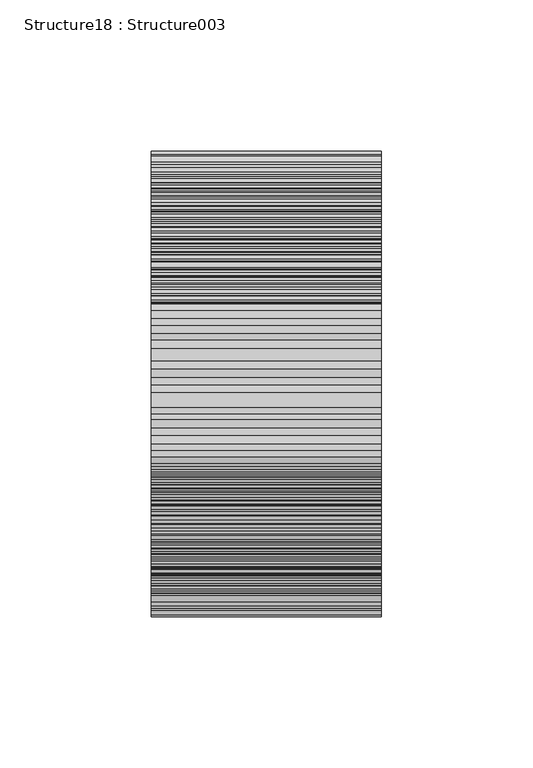
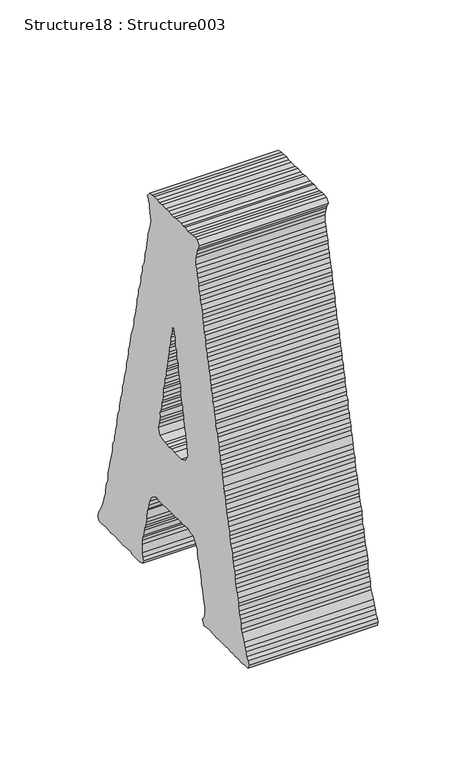
"""IFC4 building model written with IfcOpenShell, lengths in millimetres: proxy geometry, Structure18 : Structure003."""

from ifc_helpers import new_model, si_unit, frame, origin, place, context, project, spatial, polyline, outline, extrude, source, transform, mapped, element, save


def structure18_structure003_2453312d(model_context):
    return source(origin(), model_context, "Body", "SweptSolid", [
        extrude(outline(polyline([(2.1653931, 0.0), (4.9551582, -1.2470496), (7.1205514, -1.5528817), (9.8959144, -1.8705743), (12.3790002, -2.7880707), (14.2258535, -3.0939029), (17.0249376, -4.024107), (19.4987044, -4.024107), (22.2740675, -4.9534639), (24.4394606, -5.5769887), (27.2292257, -6.2005135), (29.3937717, -6.8121777), (31.8616083, -7.1180098), (33.7101559, -8.0482139), (36.8159193, -8.3540461), (38.9813125, -8.3540461), (41.7583699, -8.9775709), (43.3112516, -9.9069278), (46.4093904, -10.518592), (48.2664099, -11.1421168), (50.7384823, -11.7546283), (53.207166, -11.7546283), (55.371712, -12.3781531), (58.1614771, -13.30751), (60.6428686, -14.2250064), (63.419926, -14.2250064), (65.2676265, -15.1543633), (68.3750842, -15.7787352), (70.2219375, -15.7787352), (72.7041762, -16.7080922), (75.1770958, -17.0257848), (77.9524588, -17.6374491), (80.1322541, -18.566806), (84.4621932, -18.566806), (86.9291825, -17.9551417), (89.4029494, -17.3316169), (91.2591217, -16.40226), (93.7311941, -15.1543633), (96.2142799, -17.3316169), (96.5226536, -19.4961629), (96.5226536, -21.6615561), (95.9109893, -24.450474), (95.9109893, -26.9208521), (96.5226536, -29.70977), (96.2142799, -31.5574705), (96.5226536, -33.733877), (96.5226536, -38.6754804), (95.9109893, -41.1467056), (95.9109893, -43.6179309), (96.5226536, -46.4060017), (96.2142799, -49.1949196), (96.2142799, -53.2190266), (95.9109893, -55.996084), (96.5226536, -58.16063), (96.5226536, -60.9495479), (96.2142799, -63.114941), (95.9109893, -65.8911513), (93.4245148, -67.7507123), (91.2591217, -66.5146761), (89.0945757, -65.8911513), (87.2375562, -65.5971797), (84.4621932, -64.9736549), (79.8094783, -64.044298), (77.6457795, -64.6678227), (74.8687221, -65.279487), (69.9135639, -67.1271875), (68.3750842, -67.1271875), (65.5853191, -67.7507123), (63.1166354, -68.3742371), (60.3268703, -68.6800692), (57.8437845, -69.303594), (55.371712, -70.538783), (53.5155397, -70.538783), (50.7384823, -70.8454623), (48.2664099, -71.4689871), (46.4093904, -72.7041762), (43.6196253, -72.7041762), (41.1467056, -73.6216726), (38.9813125, -74.2451974), (36.5134759, -74.2451974), (33.7101559, -74.8695693), (31.2507912, -75.7989262), (29.085398, -76.7282832), (27.2292257, -77.0341153), (24.4394606, -77.3518079), (22.2740675, -78.2693043), (19.4987044, -78.2693043), (17.0249376, -79.1995084), (14.8510727, -79.5053406), (12.0748624, -80.1288654), (7.7322156, -81.6698865), (4.9551582, -81.6698865), (2.7906123, -82.2934113), (0.3176926, -82.9059228), (-2.4720725, -84.1529723), (-4.3282448, -84.4588045), (-6.8020116, -85.0823292), (-9.283403, -85.3881614), (-12.0604605, -86.306505), (-13.9217158, -86.9300297), (-16.7063979, -86.9300297), (-19.4826081, -87.8593867), (-21.3438635, -88.1770793), (-24.1344758, -89.1064362), (-26.5929933, -89.4004078), (-29.0752319, -89.70624), (-30.9322514, -90.3306119), (-33.4136429, -91.2599688), (-36.4982268, -91.5776615), (-38.9711464, -92.1893258), (-40.5240281, -93.1186827), (-43.3002383, -93.1186827), (-46.0908506, -93.7303469), (-48.2553966, -94.660551), (-51.0409258, -95.2840758), (-52.9021812, -95.9076006), (-55.0531722, -96.5311254), (-57.5354109, -96.5311254), (-60.6327025, -97.7544539), (-63.1013862, -98.3788259), (-65.2794871, -98.684658), (-67.7524067, -98.684658), (-69.6094262, -99.3081828), (-72.6931629, -100.2375397), (-74.5501824, -100.5433719), (-77.032421, -101.4608682), (-79.8128671, -101.4608682), (-81.9782603, -102.708765), (-84.1428062, -103.3322898), (-86.6106428, -103.3322898), (-89.386853, -103.9439541), (-92.1910202, -104.873311), (-94.3420113, -105.4849752), (-96.2032666, -106.1093472), (-98.9887958, -106.4151793), (-101.4617155, -107.3445362), (-104.2514806, -107.968061), (-106.7193172, -107.968061), (-108.8982652, -108.2857537), (-111.0492563, -109.5090822), (-113.8390214, -110.1334542), (-116.311941, -110.756979), (-118.476487, -110.756979), (-120.6503519, -111.6863359), (-125.8994818, -113.2154965), (-128.0784298, -114.1575612), (-129.9261303, -115.0869181), (-132.7116595, -116.9456319), (-134.2560694, -117.5572962), (-137.0314325, -118.4875003), (-139.2061446, -117.8639755), (-139.5136711, -114.7692254), (-139.2061446, -112.9215249), (-138.8884519, -110.1334542), (-139.5136711, -107.6622289), (-139.5136711, -104.873311), (-138.8884519, -102.4029329), (-138.8884519, -100.2375397), (-139.2061446, -97.7544539), (-139.2061446, -95.589908), (-139.5136711, -92.5070184), (-139.5136711, -90.3306119), (-139.2061446, -87.8593867), (-138.8884519, -85.0823292), (-139.5136711, -82.9059228), (-139.5136711, -75.7989262), (-138.8884519, -73.0100083), (-136.7374609, -71.7748193), (-134.8762055, -72.7041762), (-132.4083689, -73.327701), (-127.1363652, -73.327701), (-124.6634456, -73.327701), (-122.4988996, -72.7041762), (-120.6503519, -71.7748193), (-117.5437413, -71.4689871), (-115.3791954, -70.8454623), (-113.2138022, -69.9152582), (-111.0492563, -69.303594), (-108.5805725, -68.6800692), (-103.0145972, -68.0684049), (-101.4617155, -67.4448801), (-98.9887958, -66.5146761), (-95.8957401, -65.8911513), (-92.8018373, -64.3501301), (-90.9405819, -62.1847369), (-89.0928814, -58.7841547), (-89.7045457, -56.3137767), (-89.7045457, -51.3603128), (-89.386853, -48.2655627), (-89.386853, -41.7702304), (-89.7045457, -38.9813125), (-89.0928814, -36.8167665), (-89.386853, -34.3336807), (-89.7045457, -31.8633026), (-89.386853, -29.70977), (-89.0928814, -26.6031594), (-89.7045457, -24.7563061), (-90.6372913, -21.0380313), (-92.4943108, -19.1784703), (-95.8957401, -16.7080922), (-98.6719504, -16.7080922), (-101.4617155, -16.0964279), (-103.0145972, -15.1543633), (-106.0991811, -14.8485311), (-107.9697554, -13.6252026), (-110.7459657, -13.0016778), (-112.6029851, -12.6958457), (-115.0759048, -12.6958457), (-117.5437413, -11.447949), (-120.0302159, -11.1421168), (-122.4988996, -10.8244242), (-124.6634456, -9.9069278), (-127.7607372, -8.9775709), (-131.7831498, -9.283403), (-134.8762055, -10.2127599), (-136.4206154, -11.7546283), (-139.5136711, -9.9069278), (-139.2061446, -7.1180098), (-138.8884519, -4.6476317), (-138.8884519, 0.3066793), (-139.2061446, 2.7770574), (-139.2061446, 5.2601432), (-138.8884519, 7.4128287), (-139.2061446, 9.5782218), (-139.2061446, 12.6848324), (-138.8884519, 14.5316857), (-139.2061446, 17.6264358), (-138.8884519, 19.4851496), (-139.5136711, 21.9563749), (-138.8884519, 24.7452928), (-139.5136711, 27.5223502), (-139.2061446, 29.6868962), (-138.8884519, 32.169982), (-138.8884519, 34.6403601), (-136.4206154, 35.5705642), (-134.2560694, 34.9461922), (-132.7116595, 33.3933105), (-129.9261303, 32.7935068), (-128.0784298, 31.8641499), (-125.2742626, 30.6162531), (-120.6503519, 28.4635677), (-118.7797776, 27.8400429), (-115.7002768, 27.5223502), (-113.2138022, 26.9098388), (-111.0492563, 26.286314), (-109.2015558, 25.3688176), (-106.0991811, 25.0511249), (-104.2514806, 25.0511249), (-101.4617155, 24.4394607), (-98.6719504, 23.5092566), (-96.5201121, 22.5798997), (-94.3420113, 21.9563749), (-91.565801, 21.6386822), (-89.0928814, 21.3447106), (-86.9190164, 21.0388785), (-84.7629423, 19.7918289), (-81.6563317, 19.4851496), (-79.5053406, 19.167457), (-77.032421, 18.8616248), (-74.858556, 17.9322679), (-72.3856364, 17.0147715), (-69.6094262, 16.3912467), (-68.0556973, 15.7677219), (-65.5827776, 15.7677219), (-62.7980956, 14.8375178), (-60.0074833, 14.5316857), (-58.151311, 13.9081609), (-55.6783914, 12.9906645), (-53.5223172, 12.6848324), (-50.7232331, 11.7546283), (-48.2553966, 11.7546283), (-46.0908506, 11.1311035), (-43.617931, 10.5075787), (-40.8273187, 9.8840539), (-36.1949362, 8.6607254), (-33.7220165, 8.0372006), (-31.2397779, 8.0372006), (-29.0752319, 7.1069965), (-26.910686, 6.1776396), (-23.8125472, 6.1776396), (-21.9690826, 4.9543111), (-19.4826081, 4.9543111), (-16.7063979, 4.6366184), (-14.2250064, 3.4005822), (-12.0604605, 3.4005822), (-9.9094694, 2.1535326), (-6.8020116, 1.8477005), (-4.6366185, 1.8477005), (-1.8612554, 0.6125115), (0.0, 0.0), (2.1653931, 0.0)]), holes=[polyline([(-49.7947234, -33.1103522), (-49.7947234, -40.2173487), (-49.5007518, -43.0054195), (-50.1124161, -45.7943374), (-49.5007518, -47.9597306), (-49.7947234, -50.112416), (-48.2553966, -54.7600478), (-44.2423029, -56.3137767), (-41.1450113, -55.6902519), (-38.9711464, -55.0667271), (-36.8150722, -54.4423551), (-33.7220165, -54.7600478), (-31.5430685, -53.5248587), (-29.0752319, -53.2190266), (-26.910686, -52.9013339), (-24.7452928, -51.971977), (-22.2639014, -51.6661449), (-19.7909818, -51.6661449), (-17.0147715, -51.3603128), (-15.1535162, -50.4301087), (-12.6848324, -49.8065839), (-10.203441, -49.8065839), (-7.4221477, -48.5713948), (-4.6366185, -48.5713948), (-2.4720725, -47.6420379), (-0.6099699, -47.3362058), (2.4737668, -47.0185131), (4.9551582, -46.4060017), (7.423842, -45.7943374), (9.5892351, -45.4885053), (12.0748624, -45.4885053), (14.5435462, -44.2414557), (16.7089393, -43.9356236), (19.4987044, -43.9356236), (21.9563748, -43.0054195), (24.1353229, -42.3818947), (26.300716, -42.3818947), (26.6040066, -41.4643983), (24.1353229, -40.8408735), (21.6496955, -39.9115166), (19.1810118, -39.6056845), (16.4048016, -39.6056845), (14.5435462, -38.3577877), (11.7537811, -38.0519556), (9.8959144, -38.0519556), (7.423842, -36.8167665), (4.3307863, -36.5109344), (2.1653931, -36.2051023), (0.0, -35.5815775), (-2.4720725, -35.2638848), (-5.2567545, -34.3336807), (-10.203441, -34.0278486), (-12.6848324, -33.4161843), (-15.1535162, -33.1103522), (-16.7063979, -32.1809953), (-19.4826081, -32.1809953), (-21.9690826, -30.9330985), (-24.4377663, -30.9330985), (-26.5929933, -30.3214343), (-29.3920774, -30.0156022), (-31.2397779, -29.0862452), (-34.0159881, -29.0862452), (-36.8150722, -28.1568883), (-38.6627727, -28.1568883), (-41.1450113, -27.5333635), (-44.2423029, -26.9208521), (-47.9470229, -28.7804131), (-49.7947234, -33.1103522)])]), frame((-35624.0862846, 278220.7426908, 4122.0266343), z_axis=(1.0, 0.0, 1.354250045437766e-12), x_axis=(-1.354250045437766e-12, 0.0, 1.0)), (0.0, 0.0, 1.0), 76.2),
    ])


if __name__ == "__main__":
    model = new_model("IFC4")
    model_context = context("Model", 3, world=origin())
    ifc_project = project(units=[si_unit("LENGTHUNIT", "METRE", prefix="MILLI")], contexts=[model_context])
    site = spatial("IfcSite", under=ifc_project)
    building = spatial("IfcBuilding", under=site)
    placement = place(None, origin())
    structure18_structure003_shape = structure18_structure003_2453312d(model_context)
    element("IfcBuildingElementProxy", 1, Name="Structure18 : Structure003", ObjectType="Structure18 : Structure003", at=placement, inside=building, context=model_context, shape_type="MappedRepresentation", body=[
        mapped(structure18_structure003_shape, transform((0.0, 0.0, 0.0), x_axis=(1.0, 0.0, 0.0), y_axis=(0.0, 1.0, 0.0), z_axis=(0.0, 0.0, 1.0))),
    ])
    save(model, "model.ifc")

# Revit data of these elements
# Type "Structure18 : Structure003"
#   NameOverride = "Structure003"
# Element 1 (IfcBuildingElementProxy, "Structure18 : Structure003")
#   Materials on its faces: "BRUSHED ALUMINUM LETTERING"
# Materials
#   "BRUSHED ALUMINUM LETTERING": class "Unassigned", colour RGB 169 181 186, transparency 0, Cost = 0
